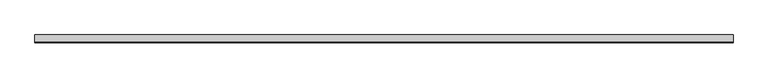
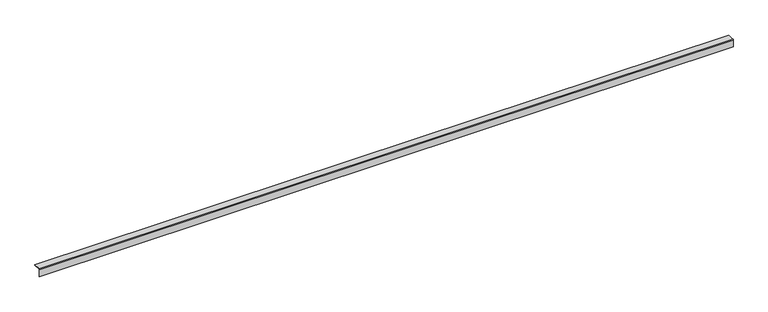
"""IFC4 building model written with IfcOpenShell, lengths in millimetres: proxy geometry, Metal profile009 3093 : Metal profile009 3093."""

from ifc_helpers import new_model, si_unit, point, frame, frame_2d, origin, place, context, project, spatial, polyline, circle_curve, trimmed, segment, composite_curve, outline, extrude, source, transform, mapped, element, save


def generic_models_aac44581(model_context):
    return source(origin(), model_context, "Body", "SweptSolid", [
        extrude(outline(composite_curve([segment(polyline([(10286.1700277, 40794.0332812), (10265.0168438, 40794.0332812), (10265.0168438, 40772.8800973), (10263.7368438, 40772.8800973), (10263.7368438, 40793.783007)]), True, "CONTINUOUS"), segment(trimmed(circle_curve(frame_2d((10264.3768438, 40794.6732812)), 1.0964434), [point((10263.7368438, 40793.783007))], [point((10265.267118, 40795.3132812))], False, "CARTESIAN"), True, "CONTINUOUS"), segment(polyline([(10265.267118, 40795.3132812), (10286.1700277, 40795.3132812), (10286.1700277, 40794.0332812)]), True, "CONTINUOUS")], self_intersect=False)), frame((3694.2883192, 0.0, 0.0), z_axis=(1.0, 0.0, 0.0), x_axis=(0.0, 1.0, 0.0)), (0.0, 0.0, 1.0), 2000.0),
    ])


if __name__ == "__main__":
    model = new_model("IFC4")
    model_context = context("Model", 3, world=origin())
    ifc_project = project(units=[si_unit("LENGTHUNIT", "METRE", prefix="MILLI")], contexts=[model_context])
    site = spatial("IfcSite", under=ifc_project)
    building = spatial("IfcBuilding", under=site)
    placement = place(None, origin())
    generic_models_shape = generic_models_aac44581(model_context)
    element("IfcBuildingElementProxy", 1, Name="Metal profile009 3093 : Metal profile009 3093", ObjectType="Metal profile009 3093 : Metal profile009 3093", at=placement, inside=building, context=model_context, shape_type="MappedRepresentation", body=[
        mapped(generic_models_shape, transform((0.0, 0.0, 0.0), x_axis=(1.0, 0.0, 0.0), y_axis=(0.0, 1.0, 0.0), z_axis=(0.0, 0.0, 1.0))),
    ])
    save(model, "model.ifc")

# Revit data of these elements
# Type "Metal profile009 3093 : Metal profile009 3093"
#   NameOverride = "Metal profile009"
# Element 1 (IfcBuildingElementProxy, "Metal profile009 3093 : Metal profile009 3093")
#   Materials on its faces: "CORNER BEAD"
# Materials
#   "CORNER BEAD": class "Unassigned", colour RGB 255 241 0, transparency 0
